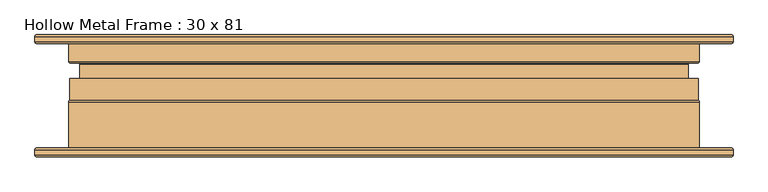
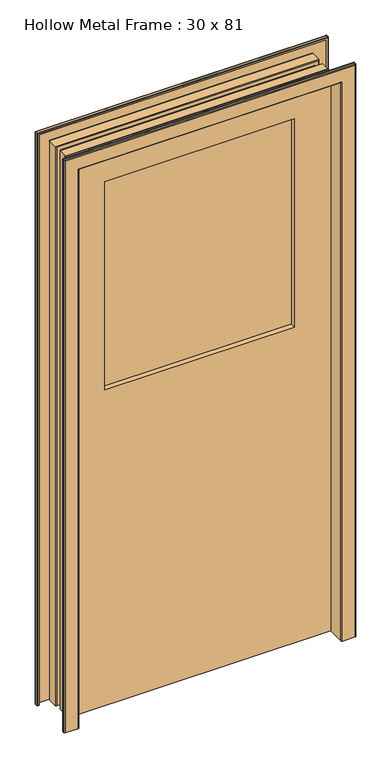
"""IFC4 building model written with IfcOpenShell, lengths in millimetres: door geometry, Hollow Metal Frame : 30 x 81."""

from ifc_helpers import new_model, si_unit, frame, origin, place, context, project, spatial, polyline, circle_curve, ellipse_curve, outline, extrude, source, transform, mapped, element, save
from ifc_brep_helpers import plane_surface, cylinder_surface, revolved_surface, advanced_brep


def hollow_metal_frame_30_x_81_1a9cdc0c(model_context):
    return source(origin(), model_context, "Body", "SolidModel", [
        extrude(outline(polyline([(330.2, 6.35), (330.2, -6.35), (-330.2, -6.35), (-330.2, 6.35), (330.2, 6.35)])), frame((0.0, 0.0, 1163.32), z_axis=(0.0, 0.0, 1.0), x_axis=(1.0, 0.0, 0.0)), (0.0, 0.0, 1.0), 767.08),
        extrude(outline(polyline([(2057.4, -457.2), (0.0, -457.2), (0.0, 457.2), (2057.4, 457.2), (2057.4, -457.2)]), holes=[polyline([(1930.4, -330.2), (1930.4, 330.2), (1163.32, 330.2), (1163.32, -330.2), (1930.4, -330.2)])]), frame((0.0, -25.4, 0.0), z_axis=(0.0, 1.0, 0.0), x_axis=(0.0, 0.0, 1.0)), (0.0, 0.0, 1.0), 50.8),
        advanced_brep(
        [(-505.42825, -76.2635, 0.0), (-500.0625, -76.2635, 0.0), (-500.0625, -77.81925, 0.0), (-505.42825, -77.81925, 0.0), (-506.44425, -78.83525, 0.0), (-506.44425, -86.36, 0.0), (-505.42825, -87.376, 0.0), (-459.77175, -87.376, 0.0), (-458.75575, -86.36, 0.0), (-458.75575, -8.98525, 0.0), (-456.184, -6.4135, 0.0), (-443.89675, -6.4135, 0.0), (-442.88075, -5.3975, 0.0), (-442.88075, 46.3931, 0.0), (-443.89675, 47.4091, 0.0), (-456.184, 47.4091, 0.0), (-458.75575, 49.98085, 0.0), (-458.75575, 86.2965, 0.0), (-459.77175, 87.3125, 0.0), (-505.42825, 87.3125, 0.0), (-506.44425, 86.2965, 0.0), (-506.44425, 78.77175, 0.0), (-505.42825, 77.75575, 0.0), (-500.0625, 77.75575, 0.0), (-500.0625, 76.2, 0.0), (-505.42825, 76.2, 0.0), (-508.0, 78.77175, 0.0), (-508.0, 86.2965, 0.0), (-505.42825, 88.86825, 0.0), (-459.77175, 88.86825, 0.0), (-457.2, 86.2965, 0.0), (-457.2, 49.98085, 0.0), (-456.184, 48.96485, 0.0), (-443.89675, 48.96485, 0.0), (-441.325, 46.3931, 0.0), (-441.325, -5.3975, 0.0), (-443.89675, -7.96925, 0.0), (-456.184, -7.96925, 0.0), (-457.2, -8.98525, 0.0), (-457.2, -86.36, 0.0), (-459.77175, -88.93175, 0.0), (-505.42825, -88.93175, 0.0), (-508.0, -86.36, 0.0), (-508.0, -78.83525, 0.0), (-508.0, -78.83525, 2108.2), (-505.42825, -76.2635, 2105.62825), (-508.0, -86.36, 2108.2), (-505.42825, -88.93175, 2105.62825), (-459.77175, -88.93175, 2059.97175), (459.77175, -88.93175, 2059.97175), (459.77175, -88.93175, 0.0), (505.42825, -88.93175, 0.0), (505.42825, -88.93175, 2105.62825), (-457.2, -86.36, 2057.4), (-457.2, -8.98525, 2057.4), (-456.184, -7.96925, 2056.384), (-443.89675, -7.96925, 2044.09675), (443.89675, -7.96925, 2044.09675), (443.89675, -7.96925, 0.0), (456.184, -7.96925, 0.0), (456.184, -7.96925, 2056.384), (-441.325, -5.3975, 2041.525), (-441.325, 46.3931, 2041.525), (-443.89675, 48.96485, 2044.09675), (-456.184, 48.96485, 2056.384), (456.184, 48.96485, 2056.384), (456.184, 48.96485, 0.0), (443.89675, 48.96485, 0.0), (443.89675, 48.96485, 2044.09675), (-457.2, 49.98085, 2057.4), (-457.2, 86.2965, 2057.4), (-459.77175, 88.86825, 2059.97175), (-505.42825, 88.86825, 2105.62825), (505.42825, 88.86825, 2105.62825), (505.42825, 88.86825, 0.0), (459.77175, 88.86825, 0.0), (459.77175, 88.86825, 2059.97175), (-508.0, 86.2965, 2108.2), (-508.0, 78.77175, 2108.2), (-505.42825, 76.2, 2105.62825), (-500.0625, 76.2, 2100.2625), (500.0625, 76.2, 2100.2625), (500.0625, 76.2, 0.0), (505.42825, 76.2, 0.0), (505.42825, 76.2, 2105.62825), (-500.0625, 77.75575, 2100.2625), (-505.42825, 77.75575, 2105.62825), (505.42825, 77.75575, 2105.62825), (505.42825, 77.75575, 0.0), (500.0625, 77.75575, 0.0), (500.0625, 77.75575, 2100.2625), (-506.44425, 78.77175, 2106.64425), (-506.44425, 86.2965, 2106.64425), (-505.42825, 87.3125, 2105.62825), (-459.77175, 87.3125, 2059.97175), (459.77175, 87.3125, 2059.97175), (459.77175, 87.3125, 0.0), (505.42825, 87.3125, 0.0), (505.42825, 87.3125, 2105.62825), (-458.75575, 86.2965, 2058.95575), (-458.75575, 49.98085, 2058.95575), (-456.184, 47.4091, 2056.384), (-443.89675, 47.4091, 2044.09675), (443.89675, 47.4091, 2044.09675), (443.89675, 47.4091, 0.0), (456.184, 47.4091, 0.0), (456.184, 47.4091, 2056.384), (-442.88075, 46.3931, 2043.08075), (-442.88075, -5.3975, 2043.08075), (-443.89675, -6.4135, 2044.09675), (-456.184, -6.4135, 2056.384), (456.184, -6.4135, 2056.384), (456.184, -6.4135, 0.0), (443.89675, -6.4135, 0.0), (443.89675, -6.4135, 2044.09675), (-458.75575, -8.98525, 2058.95575), (-458.75575, -86.36, 2058.95575), (-459.77175, -87.376, 2059.97175), (-505.42825, -87.376, 2105.62825), (505.42825, -87.376, 2105.62825), (505.42825, -87.376, 0.0), (459.77175, -87.376, 0.0), (459.77175, -87.376, 2059.97175), (-506.44425, -86.36, 2106.64425), (-506.44425, -78.83525, 2106.64425), (-505.42825, -77.81925, 2105.62825), (-500.0625, -77.81925, 2100.2625), (500.0625, -77.81925, 2100.2625), (500.0625, -77.81925, 0.0), (505.42825, -77.81925, 0.0), (505.42825, -77.81925, 2105.62825), (-500.0625, -76.2635, 2100.2625), (505.42825, -76.2635, 2105.62825), (505.42825, -76.2635, 0.0), (500.0625, -76.2635, 0.0), (500.0625, -76.2635, 2100.2625), (508.0, -78.83525, 2108.2), (508.0, -86.36, 2108.2), (457.2, -86.36, 2057.4), (457.2, -8.98525, 2057.4), (441.325, -5.3975, 2041.525), (441.325, 46.3931, 2041.525), (457.2, 49.98085, 2057.4), (457.2, 86.2965, 2057.4), (508.0, 86.2965, 2108.2), (508.0, 78.77175, 2108.2), (506.44425, 78.77175, 2106.64425), (506.44425, 86.2965, 2106.64425), (458.75575, 86.2965, 2058.95575), (458.75575, 49.98085, 2058.95575), (442.88075, 46.3931, 2043.08075), (442.88075, -5.3975, 2043.08075), (458.75575, -8.98525, 2058.95575), (458.75575, -86.36, 2058.95575), (506.44425, -86.36, 2106.64425), (506.44425, -78.83525, 2106.64425), (508.0, -78.83525, 0.0), (508.0, -86.36, 0.0), (457.2, -86.36, 0.0), (457.2, -8.98525, 0.0), (441.325, -5.3975, 0.0), (441.325, 46.3931, 0.0), (457.2, 49.98085, 0.0), (457.2, 86.2965, 0.0), (508.0, 86.2965, 0.0), (508.0, 78.77175, 0.0), (506.44425, 78.77175, 0.0), (506.44425, 86.2965, 0.0), (458.75575, 86.2965, 0.0), (458.75575, 49.98085, 0.0), (442.88075, 46.3931, 0.0), (442.88075, -5.3975, 0.0), (458.75575, -8.98525, 0.0), (458.75575, -86.36, 0.0), (506.44425, -86.36, 0.0), (506.44425, -78.83525, 0.0)],
        [
            (0, 1),
            (1, 2),
            (2, 3),
            (3, 4, circle_curve(frame((-505.42825, -78.83525, 0.0), z_axis=(0.0, 0.0, 1.0), x_axis=(0.0, 1.0, 0.0)), 1.016)),
            (4, 5),
            (5, 6, circle_curve(frame((-505.42825, -86.36, 0.0), z_axis=(0.0, 0.0, 1.0), x_axis=(0.0, 1.0, 0.0)), 1.016)),
            (6, 7),
            (7, 8, circle_curve(frame((-459.77175, -86.36, 0.0), z_axis=(0.0, 0.0, 1.0), x_axis=(0.0, 1.0, 0.0)), 1.016)),
            (8, 9),
            (9, 10, circle_curve(frame((-456.184, -8.98525, 0.0), z_axis=(0.0, 0.0, -1.0), x_axis=(0.0, 1.0, 0.0)), 2.57175)),
            (10, 11),
            (11, 12, circle_curve(frame((-443.89675, -5.3975, 0.0), z_axis=(0.0, 0.0, 1.0), x_axis=(0.0, 1.0, 0.0)), 1.016)),
            (12, 13),
            (13, 14, circle_curve(frame((-443.89675, 46.3931, 0.0), z_axis=(0.0, 0.0, 1.0), x_axis=(0.0, 1.0, 0.0)), 1.016)),
            (14, 15),
            (15, 16, circle_curve(frame((-456.184, 49.98085, 0.0), z_axis=(0.0, 0.0, -1.0), x_axis=(0.0, 1.0, 0.0)), 2.57175)),
            (16, 17),
            (17, 18, circle_curve(frame((-459.77175, 86.2965, 0.0), z_axis=(0.0, 0.0, 1.0), x_axis=(0.0, 1.0, 0.0)), 1.016)),
            (18, 19),
            (19, 20, circle_curve(frame((-505.42825, 86.2965, 0.0), z_axis=(0.0, 0.0, 1.0), x_axis=(0.0, 1.0, 0.0)), 1.016)),
            (20, 21),
            (21, 22, circle_curve(frame((-505.42825, 78.77175, 0.0), z_axis=(0.0, 0.0, 1.0), x_axis=(0.0, 1.0, 0.0)), 1.016)),
            (22, 23),
            (23, 24),
            (24, 25),
            (25, 26, circle_curve(frame((-505.42825, 78.77175, 0.0), z_axis=(0.0, 0.0, -1.0), x_axis=(0.0, 1.0, 0.0)), 2.57175)),
            (26, 27),
            (27, 28, circle_curve(frame((-505.42825, 86.2965, 0.0), z_axis=(0.0, 0.0, -1.0), x_axis=(0.0, 1.0, 0.0)), 2.57175)),
            (28, 29),
            (29, 30, circle_curve(frame((-459.77175, 86.2965, 0.0), z_axis=(0.0, 0.0, -1.0), x_axis=(0.0, 1.0, 0.0)), 2.57175)),
            (30, 31),
            (31, 32, circle_curve(frame((-456.184, 49.98085, 0.0), z_axis=(0.0, 0.0, 1.0), x_axis=(0.0, 1.0, 0.0)), 1.016)),
            (32, 33),
            (33, 34, circle_curve(frame((-443.89675, 46.3931, 0.0), z_axis=(0.0, 0.0, -1.0), x_axis=(0.0, 1.0, 0.0)), 2.57175)),
            (34, 35),
            (35, 36, circle_curve(frame((-443.89675, -5.3975, 0.0), z_axis=(0.0, 0.0, -1.0), x_axis=(0.0, 1.0, 0.0)), 2.57175)),
            (36, 37),
            (37, 38, circle_curve(frame((-456.184, -8.98525, 0.0), z_axis=(0.0, 0.0, 1.0), x_axis=(0.0, 1.0, 0.0)), 1.016)),
            (38, 39),
            (39, 40, circle_curve(frame((-459.77175, -86.36, 0.0), z_axis=(0.0, 0.0, -1.0), x_axis=(0.0, 1.0, 0.0)), 2.57175)),
            (40, 41),
            (41, 42, circle_curve(frame((-505.42825, -86.36, 0.0), z_axis=(0.0, 0.0, -1.0), x_axis=(0.0, 1.0, 0.0)), 2.57175)),
            (42, 43),
            (43, 0, circle_curve(frame((-505.42825, -78.83525, 0.0), z_axis=(0.0, 0.0, -1.0), x_axis=(0.0, 1.0, 0.0)), 2.57175)),
            (43, 44),
            (44, 45, ellipse_curve(frame((-505.42825, -78.83525, 2105.62825), z_axis=(-0.7071067811865475, 0.0, -0.7071067811865475), x_axis=(0.7071067811865474, 0.0, -0.7071067811865476)), 3.6370037, 2.57175)),
            (45, 0),
            (42, 46),
            (46, 44),
            (41, 47),
            (47, 46, ellipse_curve(frame((-505.42825, -86.36, 2105.62825), z_axis=(-0.7071067811865475, 0.0, -0.7071067811865475), x_axis=(0.7071067811865474, 0.0, -0.7071067811865476)), 3.6370037, 2.57175)),
            (40, 48),
            (48, 49),
            (49, 50),
            (50, 51),
            (51, 52),
            (52, 47),
            (39, 53),
            (53, 48, ellipse_curve(frame((-459.77175, -86.36, 2059.97175), z_axis=(-0.7071067811865475, 0.0, -0.7071067811865475), x_axis=(0.7071067811865474, 0.0, -0.7071067811865476)), 3.6370037, 2.57175)),
            (38, 54),
            (54, 53),
            (37, 55),
            (55, 54, ellipse_curve(frame((-456.184, -8.98525, 2056.384), z_axis=(0.7071067811865475, 0.0, 0.7071067811865475), x_axis=(-0.7071067811865474, 0.0, 0.7071067811865476)), 1.436841, 1.016)),
            (36, 56),
            (56, 57),
            (57, 58),
            (58, 59),
            (59, 60),
            (60, 55),
            (35, 61),
            (61, 56, ellipse_curve(frame((-443.89675, -5.3975, 2044.09675), z_axis=(-0.7071067811865475, 0.0, -0.7071067811865475), x_axis=(0.7071067811865474, 0.0, -0.7071067811865476)), 3.6370037, 2.57175)),
            (34, 62),
            (62, 61),
            (33, 63),
            (63, 62, ellipse_curve(frame((-443.89675, 46.3931, 2044.09675), z_axis=(-0.7071067811865475, 0.0, -0.7071067811865475), x_axis=(0.7071067811865474, 0.0, -0.7071067811865476)), 3.6370037, 2.57175)),
            (32, 64),
            (64, 65),
            (65, 66),
            (66, 67),
            (67, 68),
            (68, 63),
            (31, 69),
            (69, 64, ellipse_curve(frame((-456.184, 49.98085, 2056.384), z_axis=(0.7071067811865475, 0.0, 0.7071067811865475), x_axis=(-0.7071067811865474, 0.0, 0.7071067811865476)), 1.436841, 1.016)),
            (30, 70),
            (70, 69),
            (29, 71),
            (71, 70, ellipse_curve(frame((-459.77175, 86.2965, 2059.97175), z_axis=(-0.7071067811865475, 0.0, -0.7071067811865475), x_axis=(0.7071067811865474, 0.0, -0.7071067811865476)), 3.6370037, 2.57175)),
            (28, 72),
            (72, 73),
            (73, 74),
            (74, 75),
            (75, 76),
            (76, 71),
            (27, 77),
            (77, 72, ellipse_curve(frame((-505.42825, 86.2965, 2105.62825), z_axis=(-0.7071067811865475, 0.0, -0.7071067811865475), x_axis=(0.7071067811865474, 0.0, -0.7071067811865476)), 3.6370037, 2.57175)),
            (26, 78),
            (78, 77),
            (25, 79),
            (79, 78, ellipse_curve(frame((-505.42825, 78.77175, 2105.62825), z_axis=(-0.7071067811865475, 0.0, -0.7071067811865475), x_axis=(0.7071067811865474, 0.0, -0.7071067811865476)), 3.6370037, 2.57175)),
            (24, 80),
            (80, 81),
            (81, 82),
            (82, 83),
            (83, 84),
            (84, 79),
            (23, 85),
            (85, 80),
            (22, 86),
            (86, 87),
            (87, 88),
            (88, 89),
            (89, 90),
            (90, 85),
            (21, 91),
            (91, 86, ellipse_curve(frame((-505.42825, 78.77175, 2105.62825), z_axis=(0.7071067811865475, 0.0, 0.7071067811865475), x_axis=(-0.7071067811865474, 0.0, 0.7071067811865476)), 1.436841, 1.016)),
            (20, 92),
            (92, 91),
            (19, 93),
            (93, 92, ellipse_curve(frame((-505.42825, 86.2965, 2105.62825), z_axis=(0.7071067811865475, 0.0, 0.7071067811865475), x_axis=(-0.7071067811865474, 0.0, 0.7071067811865476)), 1.436841, 1.016)),
            (18, 94),
            (94, 95),
            (95, 96),
            (96, 97),
            (97, 98),
            (98, 93),
            (17, 99),
            (99, 94, ellipse_curve(frame((-459.77175, 86.2965, 2059.97175), z_axis=(0.7071067811865475, 0.0, 0.7071067811865475), x_axis=(-0.7071067811865474, 0.0, 0.7071067811865476)), 1.436841, 1.016)),
            (16, 100),
            (100, 99),
            (15, 101),
            (101, 100, ellipse_curve(frame((-456.184, 49.98085, 2056.384), z_axis=(-0.7071067811865475, 0.0, -0.7071067811865475), x_axis=(0.7071067811865474, 0.0, -0.7071067811865476)), 3.6370037, 2.57175)),
            (14, 102),
            (102, 103),
            (103, 104),
            (104, 105),
            (105, 106),
            (106, 101),
            (13, 107),
            (107, 102, ellipse_curve(frame((-443.89675, 46.3931, 2044.09675), z_axis=(0.7071067811865475, 0.0, 0.7071067811865475), x_axis=(-0.7071067811865474, 0.0, 0.7071067811865476)), 1.436841, 1.016)),
            (12, 108),
            (108, 107),
            (11, 109),
            (109, 108, ellipse_curve(frame((-443.89675, -5.3975, 2044.09675), z_axis=(0.7071067811865475, 0.0, 0.7071067811865475), x_axis=(-0.7071067811865474, 0.0, 0.7071067811865476)), 1.436841, 1.016)),
            (10, 110),
            (110, 111),
            (111, 112),
            (112, 113),
            (113, 114),
            (114, 109),
            (9, 115),
            (115, 110, ellipse_curve(frame((-456.184, -8.98525, 2056.384), z_axis=(-0.7071067811865475, 0.0, -0.7071067811865475), x_axis=(0.7071067811865474, 0.0, -0.7071067811865476)), 3.6370037, 2.57175)),
            (8, 116),
            (116, 115),
            (7, 117),
            (117, 116, ellipse_curve(frame((-459.77175, -86.36, 2059.97175), z_axis=(0.7071067811865475, 0.0, 0.7071067811865475), x_axis=(-0.7071067811865474, 0.0, 0.7071067811865476)), 1.436841, 1.016)),
            (6, 118),
            (118, 119),
            (119, 120),
            (120, 121),
            (121, 122),
            (122, 117),
            (5, 123),
            (123, 118, ellipse_curve(frame((-505.42825, -86.36, 2105.62825), z_axis=(0.7071067811865475, 0.0, 0.7071067811865475), x_axis=(-0.7071067811865474, 0.0, 0.7071067811865476)), 1.436841, 1.016)),
            (4, 124),
            (124, 123),
            (3, 125),
            (125, 124, ellipse_curve(frame((-505.42825, -78.83525, 2105.62825), z_axis=(0.7071067811865475, 0.0, 0.7071067811865475), x_axis=(-0.7071067811865474, 0.0, 0.7071067811865476)), 1.436841, 1.016)),
            (2, 126),
            (126, 127),
            (127, 128),
            (128, 129),
            (129, 130),
            (130, 125),
            (1, 131),
            (131, 126),
            (45, 132),
            (132, 133),
            (133, 134),
            (134, 135),
            (135, 131),
            (44, 136),
            (136, 132, ellipse_curve(frame((505.42825, -78.83525, 2105.62825), z_axis=(-0.7071067811865475, 0.0, 0.7071067811865475), x_axis=(-0.7071067811865476, 0.0, -0.7071067811865474)), 3.6370037, 2.57175)),
            (46, 137),
            (137, 136),
            (52, 137, ellipse_curve(frame((505.42825, -86.36, 2105.62825), z_axis=(-0.7071067811865475, 0.0, 0.7071067811865475), x_axis=(-0.7071067811865476, 0.0, -0.7071067811865474)), 3.6370037, 2.57175)),
            (53, 138),
            (138, 49, ellipse_curve(frame((459.77175, -86.36, 2059.97175), z_axis=(-0.7071067811865475, 0.0, 0.7071067811865475), x_axis=(-0.7071067811865476, 0.0, -0.7071067811865474)), 3.6370037, 2.57175)),
            (54, 139),
            (139, 138),
            (60, 139, ellipse_curve(frame((456.184, -8.98525, 2056.384), z_axis=(0.7071067811865475, 0.0, -0.7071067811865475), x_axis=(0.7071067811865476, 0.0, 0.7071067811865474)), 1.436841, 1.016)),
            (61, 140),
            (140, 57, ellipse_curve(frame((443.89675, -5.3975, 2044.09675), z_axis=(-0.7071067811865475, 0.0, 0.7071067811865475), x_axis=(-0.7071067811865476, 0.0, -0.7071067811865474)), 3.6370037, 2.57175)),
            (62, 141),
            (141, 140),
            (68, 141, ellipse_curve(frame((443.89675, 46.3931, 2044.09675), z_axis=(-0.7071067811865475, 0.0, 0.7071067811865475), x_axis=(-0.7071067811865476, 0.0, -0.7071067811865474)), 3.6370037, 2.57175)),
            (69, 142),
            (142, 65, ellipse_curve(frame((456.184, 49.98085, 2056.384), z_axis=(0.7071067811865475, 0.0, -0.7071067811865475), x_axis=(0.7071067811865476, 0.0, 0.7071067811865474)), 1.436841, 1.016)),
            (70, 143),
            (143, 142),
            (76, 143, ellipse_curve(frame((459.77175, 86.2965, 2059.97175), z_axis=(-0.7071067811865475, 0.0, 0.7071067811865475), x_axis=(-0.7071067811865476, 0.0, -0.7071067811865474)), 3.6370037, 2.57175)),
            (77, 144),
            (144, 73, ellipse_curve(frame((505.42825, 86.2965, 2105.62825), z_axis=(-0.7071067811865475, 0.0, 0.7071067811865475), x_axis=(-0.7071067811865476, 0.0, -0.7071067811865474)), 3.6370037, 2.57175)),
            (78, 145),
            (145, 144),
            (84, 145, ellipse_curve(frame((505.42825, 78.77175, 2105.62825), z_axis=(-0.7071067811865475, 0.0, 0.7071067811865475), x_axis=(-0.7071067811865476, 0.0, -0.7071067811865474)), 3.6370037, 2.57175)),
            (90, 81),
            (91, 146),
            (146, 87, ellipse_curve(frame((505.42825, 78.77175, 2105.62825), z_axis=(0.7071067811865475, 0.0, -0.7071067811865475), x_axis=(0.7071067811865476, 0.0, 0.7071067811865474)), 1.436841, 1.016)),
            (92, 147),
            (147, 146),
            (98, 147, ellipse_curve(frame((505.42825, 86.2965, 2105.62825), z_axis=(0.7071067811865475, 0.0, -0.7071067811865475), x_axis=(0.7071067811865476, 0.0, 0.7071067811865474)), 1.436841, 1.016)),
            (99, 148),
            (148, 95, ellipse_curve(frame((459.77175, 86.2965, 2059.97175), z_axis=(0.7071067811865475, 0.0, -0.7071067811865475), x_axis=(0.7071067811865476, 0.0, 0.7071067811865474)), 1.436841, 1.016)),
            (100, 149),
            (149, 148),
            (106, 149, ellipse_curve(frame((456.184, 49.98085, 2056.384), z_axis=(-0.7071067811865475, 0.0, 0.7071067811865475), x_axis=(-0.7071067811865476, 0.0, -0.7071067811865474)), 3.6370037, 2.57175)),
            (107, 150),
            (150, 103, ellipse_curve(frame((443.89675, 46.3931, 2044.09675), z_axis=(0.7071067811865475, 0.0, -0.7071067811865475), x_axis=(0.7071067811865476, 0.0, 0.7071067811865474)), 1.436841, 1.016)),
            (108, 151),
            (151, 150),
            (114, 151, ellipse_curve(frame((443.89675, -5.3975, 2044.09675), z_axis=(0.7071067811865475, 0.0, -0.7071067811865475), x_axis=(0.7071067811865476, 0.0, 0.7071067811865474)), 1.436841, 1.016)),
            (115, 152),
            (152, 111, ellipse_curve(frame((456.184, -8.98525, 2056.384), z_axis=(-0.7071067811865475, 0.0, 0.7071067811865475), x_axis=(-0.7071067811865476, 0.0, -0.7071067811865474)), 3.6370037, 2.57175)),
            (116, 153),
            (153, 152),
            (122, 153, ellipse_curve(frame((459.77175, -86.36, 2059.97175), z_axis=(0.7071067811865475, 0.0, -0.7071067811865475), x_axis=(0.7071067811865476, 0.0, 0.7071067811865474)), 1.436841, 1.016)),
            (123, 154),
            (154, 119, ellipse_curve(frame((505.42825, -86.36, 2105.62825), z_axis=(0.7071067811865475, 0.0, -0.7071067811865475), x_axis=(0.7071067811865476, 0.0, 0.7071067811865474)), 1.436841, 1.016)),
            (124, 155),
            (155, 154),
            (130, 155, ellipse_curve(frame((505.42825, -78.83525, 2105.62825), z_axis=(0.7071067811865475, 0.0, -0.7071067811865475), x_axis=(0.7071067811865476, 0.0, 0.7071067811865474)), 1.436841, 1.016)),
            (135, 127),
            (133, 156, circle_curve(frame((505.42825, -78.83525, 0.0), z_axis=(0.0, 0.0, -1.0), x_axis=(0.0, 1.0, 0.0)), 2.57175)),
            (156, 157),
            (157, 51, circle_curve(frame((505.42825, -86.36, 0.0), z_axis=(0.0, 0.0, -1.0), x_axis=(0.0, 1.0, 0.0)), 2.57175)),
            (50, 158, circle_curve(frame((459.77175, -86.36, 0.0), z_axis=(0.0, 0.0, -1.0), x_axis=(0.0, 1.0, 0.0)), 2.57175)),
            (158, 159),
            (159, 59, circle_curve(frame((456.184, -8.98525, 0.0), z_axis=(0.0, 0.0, 1.0), x_axis=(0.0, 1.0, 0.0)), 1.016)),
            (58, 160, circle_curve(frame((443.89675, -5.3975, 0.0), z_axis=(0.0, 0.0, -1.0), x_axis=(0.0, 1.0, 0.0)), 2.57175)),
            (160, 161),
            (161, 67, circle_curve(frame((443.89675, 46.3931, 0.0), z_axis=(0.0, 0.0, -1.0), x_axis=(0.0, 1.0, 0.0)), 2.57175)),
            (66, 162, circle_curve(frame((456.184, 49.98085, 0.0), z_axis=(0.0, 0.0, 1.0), x_axis=(0.0, 1.0, 0.0)), 1.016)),
            (162, 163),
            (163, 75, circle_curve(frame((459.77175, 86.2965, 0.0), z_axis=(0.0, 0.0, -1.0), x_axis=(0.0, 1.0, 0.0)), 2.57175)),
            (74, 164, circle_curve(frame((505.42825, 86.2965, 0.0), z_axis=(0.0, 0.0, -1.0), x_axis=(0.0, 1.0, 0.0)), 2.57175)),
            (164, 165),
            (165, 83, circle_curve(frame((505.42825, 78.77175, 0.0), z_axis=(0.0, 0.0, -1.0), x_axis=(0.0, 1.0, 0.0)), 2.57175)),
            (82, 89),
            (88, 166, circle_curve(frame((505.42825, 78.77175, 0.0), z_axis=(0.0, 0.0, 1.0), x_axis=(0.0, 1.0, 0.0)), 1.016)),
            (166, 167),
            (167, 97, circle_curve(frame((505.42825, 86.2965, 0.0), z_axis=(0.0, 0.0, 1.0), x_axis=(0.0, 1.0, 0.0)), 1.016)),
            (96, 168, circle_curve(frame((459.77175, 86.2965, 0.0), z_axis=(0.0, 0.0, 1.0), x_axis=(0.0, 1.0, 0.0)), 1.016)),
            (168, 169),
            (169, 105, circle_curve(frame((456.184, 49.98085, 0.0), z_axis=(0.0, 0.0, -1.0), x_axis=(0.0, 1.0, 0.0)), 2.57175)),
            (104, 170, circle_curve(frame((443.89675, 46.3931, 0.0), z_axis=(0.0, 0.0, 1.0), x_axis=(0.0, 1.0, 0.0)), 1.016)),
            (170, 171),
            (171, 113, circle_curve(frame((443.89675, -5.3975, 0.0), z_axis=(0.0, 0.0, 1.0), x_axis=(0.0, 1.0, 0.0)), 1.016)),
            (112, 172, circle_curve(frame((456.184, -8.98525, 0.0), z_axis=(0.0, 0.0, -1.0), x_axis=(0.0, 1.0, 0.0)), 2.57175)),
            (172, 173),
            (173, 121, circle_curve(frame((459.77175, -86.36, 0.0), z_axis=(0.0, 0.0, 1.0), x_axis=(0.0, 1.0, 0.0)), 1.016)),
            (120, 174, circle_curve(frame((505.42825, -86.36, 0.0), z_axis=(0.0, 0.0, 1.0), x_axis=(0.0, 1.0, 0.0)), 1.016)),
            (174, 175),
            (175, 129, circle_curve(frame((505.42825, -78.83525, 0.0), z_axis=(0.0, 0.0, 1.0), x_axis=(0.0, 1.0, 0.0)), 1.016)),
            (128, 134),
            (136, 156),
            (137, 157),
            (138, 158),
            (139, 159),
            (140, 160),
            (141, 161),
            (142, 162),
            (143, 163),
            (144, 164),
            (145, 165),
            (146, 166),
            (147, 167),
            (148, 168),
            (149, 169),
            (150, 170),
            (151, 171),
            (152, 172),
            (153, 173),
            (154, 174),
            (155, 175),
        ],
        [
            plane_surface(frame((-468.3125, 76.2, 0.0), z_axis=(0.0, 0.0, -1.0), x_axis=(1.0, 0.0, 0.0))),
            cylinder_surface(frame((-505.42825, -78.83525, 0.0), z_axis=(0.0, 0.0, -1.0), x_axis=(0.0, 1.0, 0.0)), 2.57175),
            plane_surface(frame((-508.0, -78.83525, 0.0), z_axis=(-1.0, 0.0, 0.0), x_axis=(0.0, 0.0, 1.0))),
            cylinder_surface(frame((-505.42825, -86.36, 0.0), z_axis=(0.0, 0.0, -1.0), x_axis=(0.0, 1.0, 0.0)), 2.57175),
            plane_surface(frame((-505.42825, -88.93175, 0.0), z_axis=(0.0, -1.0, 0.0), x_axis=(0.0, 0.0, 1.0))),
            cylinder_surface(frame((-459.77175, -86.36, 0.0), z_axis=(0.0, 0.0, -1.0), x_axis=(0.0, 1.0, 0.0)), 2.57175),
            plane_surface(frame((-457.2, -86.36, 0.0), z_axis=(1.0, 0.0, 0.0), x_axis=(0.0, 0.0, 1.0))),
            revolved_surface(polyline([(-456.184, -7.969250000000001, 2057.400000014587), (-456.184, -7.969250000000001, 0.0)]), (-456.184, -8.98525, 0.0), (0.0, 0.0, 1.0)),
            plane_surface(frame((-456.184, -7.96925, 0.0), z_axis=(0.0, -1.0, 0.0), x_axis=(0.0, 0.0, 1.0))),
            cylinder_surface(frame((-443.89675, -5.3975, 0.0), z_axis=(0.0, 0.0, -1.0), x_axis=(0.0, 1.0, 0.0)), 2.57175),
            plane_surface(frame((-441.325, -5.3975, 0.0), z_axis=(1.0, 0.0, 0.0), x_axis=(0.0, 0.0, 1.0))),
            cylinder_surface(frame((-443.89675, 46.3931, 0.0), z_axis=(0.0, 0.0, -1.0), x_axis=(0.0, 1.0, 0.0)), 2.57175),
            plane_surface(frame((-443.89675, 48.96485, 0.0), z_axis=(0.0, 1.0, 0.0), x_axis=(0.0, 0.0, 1.0))),
            revolved_surface(polyline([(-456.184, 50.996849999999995, 2057.400000014587), (-456.184, 50.996849999999995, 0.0)]), (-456.184, 49.98085, 0.0), (0.0, 0.0, 1.0)),
            plane_surface(frame((-457.2, 49.98085, 0.0), z_axis=(1.0, 0.0, 0.0), x_axis=(0.0, 0.0, 1.0))),
            cylinder_surface(frame((-459.77175, 86.2965, 0.0), z_axis=(0.0, 0.0, -1.0), x_axis=(0.0, 1.0, 0.0)), 2.57175),
            plane_surface(frame((-459.77175, 88.86825, 0.0), z_axis=(0.0, 1.0, 0.0), x_axis=(0.0, 0.0, 1.0))),
            cylinder_surface(frame((-505.42825, 86.2965, 0.0), z_axis=(0.0, 0.0, -1.0), x_axis=(0.0, 1.0, 0.0)), 2.57175),
            plane_surface(frame((-508.0, 86.2965, 0.0), z_axis=(-1.0, 0.0, 0.0), x_axis=(0.0, 0.0, 1.0))),
            cylinder_surface(frame((-505.42825, 78.77175, 0.0), z_axis=(0.0, 0.0, -1.0), x_axis=(0.0, 1.0, 0.0)), 2.57175),
            plane_surface(frame((-505.42825, 76.2, 0.0), z_axis=(0.0, -1.0, 0.0), x_axis=(0.0, 0.0, 1.0))),
            plane_surface(frame((-500.0625, 76.2, 0.0), z_axis=(1.0, 0.0, 0.0), x_axis=(0.0, 0.0, 1.0))),
            plane_surface(frame((-500.0625, 77.75575, 0.0), z_axis=(0.0, 1.0, 0.0), x_axis=(0.0, 0.0, 1.0))),
            revolved_surface(polyline([(-505.42825, 79.78775, 2106.644250014587), (-505.42825, 79.78775, 0.0)]), (-505.42825, 78.77175, 0.0), (0.0, 0.0, 1.0)),
            plane_surface(frame((-506.44425, 78.77175, 0.0), z_axis=(1.0, 0.0, 0.0), x_axis=(0.0, 0.0, 1.0))),
            revolved_surface(polyline([(-505.42825, 87.3125, 2106.644250014587), (-505.42825, 87.3125, 0.0)]), (-505.42825, 86.2965, 0.0), (0.0, 0.0, 1.0)),
            plane_surface(frame((-505.42825, 87.3125, 0.0), z_axis=(0.0, -1.0, 0.0), x_axis=(0.0, 0.0, 1.0))),
            revolved_surface(polyline([(-459.77175, 87.3125, 2060.987750014587), (-459.77175, 87.3125, 0.0)]), (-459.77175, 86.2965, 0.0), (0.0, 0.0, 1.0)),
            plane_surface(frame((-458.75575, 86.2965, 0.0), z_axis=(-1.0, 0.0, 0.0), x_axis=(0.0, 0.0, 1.0))),
            cylinder_surface(frame((-456.184, 49.98085, 0.0), z_axis=(0.0, 0.0, -1.0), x_axis=(0.0, 1.0, 0.0)), 2.57175),
            plane_surface(frame((-456.184, 47.4091, 0.0), z_axis=(0.0, -1.0, 0.0), x_axis=(0.0, 0.0, 1.0))),
            revolved_surface(polyline([(-443.89675, 47.409099999999995, 2045.1127500145867), (-443.89675, 47.409099999999995, 0.0)]), (-443.89675, 46.3931, 0.0), (0.0, 0.0, 1.0)),
            plane_surface(frame((-442.88075, 46.3931, 0.0), z_axis=(-1.0, 0.0, 0.0), x_axis=(0.0, 0.0, 1.0))),
            revolved_surface(polyline([(-443.89675, -4.3815, 2045.1127500145867), (-443.89675, -4.3815, 0.0)]), (-443.89675, -5.3975, 0.0), (0.0, 0.0, 1.0)),
            plane_surface(frame((-443.89675, -6.4135, 0.0), z_axis=(0.0, 1.0, 0.0), x_axis=(0.0, 0.0, 1.0))),
            cylinder_surface(frame((-456.184, -8.98525, 0.0), z_axis=(0.0, 0.0, -1.0), x_axis=(0.0, 1.0, 0.0)), 2.57175),
            plane_surface(frame((-458.75575, -8.98525, 0.0), z_axis=(-1.0, 0.0, 0.0), x_axis=(0.0, 0.0, 1.0))),
            revolved_surface(polyline([(-459.77175, -85.344, 2060.987750014587), (-459.77175, -85.344, 0.0)]), (-459.77175, -86.36, 0.0), (0.0, 0.0, 1.0)),
            plane_surface(frame((-459.77175, -87.376, 0.0), z_axis=(0.0, 1.0, 0.0), x_axis=(0.0, 0.0, 1.0))),
            revolved_surface(polyline([(-505.42825, -85.344, 2106.644250014587), (-505.42825, -85.344, 0.0)]), (-505.42825, -86.36, 0.0), (0.0, 0.0, 1.0)),
            plane_surface(frame((-506.44425, -86.36, 0.0), z_axis=(1.0, 0.0, 0.0), x_axis=(0.0, 0.0, 1.0))),
            revolved_surface(polyline([(-505.42825, -77.81925, 2106.644250014587), (-505.42825, -77.81925, 0.0)]), (-505.42825, -78.83525, 0.0), (0.0, 0.0, 1.0)),
            plane_surface(frame((-505.42825, -77.81925, 0.0), z_axis=(0.0, -1.0, 0.0), x_axis=(0.0, 0.0, 1.0))),
            plane_surface(frame((-500.0625, -77.81925, 0.0), z_axis=(1.0, 0.0, 0.0), x_axis=(0.0, 0.0, 1.0))),
            plane_surface(frame((-500.0625, -76.2635, 0.0), z_axis=(0.0, 1.0, 0.0), x_axis=(0.0, 0.0, 1.0))),
            cylinder_surface(frame((-468.3125, -78.83525, 2105.62825), z_axis=(-1.0, 0.0, 0.0), x_axis=(0.0, 1.0, 0.0)), 2.57175),
            plane_surface(frame((-508.0, -78.83525, 2108.2), z_axis=(0.0, 0.0, 1.0), x_axis=(1.0, 0.0, 0.0))),
            cylinder_surface(frame((-468.3125, -86.36, 2105.62825), z_axis=(-1.0, 0.0, 0.0), x_axis=(0.0, 1.0, 0.0)), 2.57175),
            cylinder_surface(frame((-468.3125, -86.36, 2059.97175), z_axis=(-1.0, 0.0, 0.0), x_axis=(0.0, 1.0, 0.0)), 2.57175),
            plane_surface(frame((-457.2, -86.36, 2057.4), z_axis=(0.0, 0.0, -1.0), x_axis=(1.0, 0.0, 0.0))),
            revolved_surface(polyline([(457.20000001458686, -7.969250000000001, 2056.384), (-457.20000001458686, -7.969250000000001, 2056.384)]), (-468.3125, -8.98525, 2056.384), (1.0, 0.0, 0.0)),
            cylinder_surface(frame((-468.3125, -5.3975, 2044.09675), z_axis=(-1.0, 0.0, 0.0), x_axis=(0.0, 1.0, 0.0)), 2.57175),
            plane_surface(frame((-441.325, -5.3975, 2041.525), z_axis=(0.0, 0.0, -1.0), x_axis=(1.0, 0.0, 0.0))),
            cylinder_surface(frame((-468.3125, 46.3931, 2044.09675), z_axis=(-1.0, 0.0, 0.0), x_axis=(0.0, 1.0, 0.0)), 2.57175),
            revolved_surface(polyline([(457.20000001458686, 50.996849999999995, 2056.384), (-457.20000001458686, 50.996849999999995, 2056.384)]), (-468.3125, 49.98085, 2056.384), (1.0, 0.0, 0.0)),
            plane_surface(frame((-457.2, 49.98085, 2057.4), z_axis=(0.0, 0.0, -1.0), x_axis=(1.0, 0.0, 0.0))),
            cylinder_surface(frame((-468.3125, 86.2965, 2059.97175), z_axis=(-1.0, 0.0, 0.0), x_axis=(0.0, 1.0, 0.0)), 2.57175),
            cylinder_surface(frame((-468.3125, 86.2965, 2105.62825), z_axis=(-1.0, 0.0, 0.0), x_axis=(0.0, 1.0, 0.0)), 2.57175),
            plane_surface(frame((-508.0, 86.2965, 2108.2), z_axis=(0.0, 0.0, 1.0), x_axis=(1.0, 0.0, 0.0))),
            cylinder_surface(frame((-468.3125, 78.77175, 2105.62825), z_axis=(-1.0, 0.0, 0.0), x_axis=(0.0, 1.0, 0.0)), 2.57175),
            plane_surface(frame((-500.0625, 76.2, 2100.2625), z_axis=(0.0, 0.0, -1.0), x_axis=(1.0, 0.0, 0.0))),
            revolved_surface(polyline([(506.4442500145868, 79.78775, 2105.62825), (-506.4442500145868, 79.78775, 2105.62825)]), (-468.3125, 78.77175, 2105.62825), (1.0, 0.0, 0.0)),
            plane_surface(frame((-506.44425, 78.77175, 2106.64425), z_axis=(0.0, 0.0, -1.0), x_axis=(1.0, 0.0, 0.0))),
            revolved_surface(polyline([(506.4442500145868, 87.3125, 2105.62825), (-506.4442500145868, 87.3125, 2105.62825)]), (-468.3125, 86.2965, 2105.62825), (1.0, 0.0, 0.0)),
            revolved_surface(polyline([(460.7877500145869, 87.3125, 2059.97175), (-460.78775001458683, 87.3125, 2059.97175)]), (-468.3125, 86.2965, 2059.97175), (1.0, 0.0, 0.0)),
            plane_surface(frame((-458.75575, 86.2965, 2058.95575), z_axis=(0.0, 0.0, 1.0), x_axis=(1.0, 0.0, 0.0))),
            cylinder_surface(frame((-468.3125, 49.98085, 2056.384), z_axis=(-1.0, 0.0, 0.0), x_axis=(0.0, 1.0, 0.0)), 2.57175),
            revolved_surface(polyline([(444.9127500145869, 47.409099999999995, 2044.09675), (-444.91275001458683, 47.409099999999995, 2044.09675)]), (-468.3125, 46.3931, 2044.09675), (1.0, 0.0, 0.0)),
            plane_surface(frame((-442.88075, 46.3931, 2043.08075), z_axis=(0.0, 0.0, 1.0), x_axis=(1.0, 0.0, 0.0))),
            revolved_surface(polyline([(444.9127500145869, -4.3815, 2044.09675), (-444.91275001458683, -4.3815, 2044.09675)]), (-468.3125, -5.3975, 2044.09675), (1.0, 0.0, 0.0)),
            cylinder_surface(frame((-468.3125, -8.98525, 2056.384), z_axis=(-1.0, 0.0, 0.0), x_axis=(0.0, 1.0, 0.0)), 2.57175),
            plane_surface(frame((-458.75575, -8.98525, 2058.95575), z_axis=(0.0, 0.0, 1.0), x_axis=(1.0, 0.0, 0.0))),
            revolved_surface(polyline([(460.7877500145869, -85.344, 2059.97175), (-460.78775001458683, -85.344, 2059.97175)]), (-468.3125, -86.36, 2059.97175), (1.0, 0.0, 0.0)),
            revolved_surface(polyline([(506.4442500145868, -85.344, 2105.62825), (-506.4442500145868, -85.344, 2105.62825)]), (-468.3125, -86.36, 2105.62825), (1.0, 0.0, 0.0)),
            plane_surface(frame((-506.44425, -86.36, 2106.64425), z_axis=(0.0, 0.0, -1.0), x_axis=(1.0, 0.0, 0.0))),
            revolved_surface(polyline([(506.4442500145868, -77.81925, 2105.62825), (-506.4442500145868, -77.81925, 2105.62825)]), (-468.3125, -78.83525, 2105.62825), (1.0, 0.0, 0.0)),
            plane_surface(frame((-500.0625, -77.81925, 2100.2625), z_axis=(0.0, 0.0, -1.0), x_axis=(1.0, 0.0, 0.0))),
            plane_surface(frame((468.3125, 76.2, 0.0), z_axis=(0.0, 0.0, -1.0), x_axis=(-1.0, 0.0, 0.0))),
            cylinder_surface(frame((505.42825, -78.83525, 2068.5125), z_axis=(0.0, 0.0, 1.0), x_axis=(0.0, 1.0, 0.0)), 2.57175),
            plane_surface(frame((508.0, -78.83525, 2108.2), z_axis=(1.0, 0.0, 0.0), x_axis=(0.0, 0.0, -1.0))),
            cylinder_surface(frame((505.42825, -86.36, 2068.5125), z_axis=(0.0, 0.0, 1.0), x_axis=(0.0, 1.0, 0.0)), 2.57175),
            cylinder_surface(frame((459.77175, -86.36, 2068.5125), z_axis=(0.0, 0.0, 1.0), x_axis=(0.0, 1.0, 0.0)), 2.57175),
            plane_surface(frame((457.2, -86.36, 2057.4), z_axis=(-1.0, 0.0, 0.0), x_axis=(0.0, 0.0, -1.0))),
            revolved_surface(polyline([(456.184, -7.969250000000001, 0.0), (456.184, -7.969250000000001, 2057.400000014587)]), (456.184, -8.98525, 2068.5125), (0.0, 0.0, -1.0)),
            cylinder_surface(frame((443.89675, -5.3975, 2068.5125), z_axis=(0.0, 0.0, 1.0), x_axis=(0.0, 1.0, 0.0)), 2.57175),
            plane_surface(frame((441.325, -5.3975, 2041.525), z_axis=(-1.0, 0.0, 0.0), x_axis=(0.0, 0.0, -1.0))),
            cylinder_surface(frame((443.89675, 46.3931, 2068.5125), z_axis=(0.0, 0.0, 1.0), x_axis=(0.0, 1.0, 0.0)), 2.57175),
            revolved_surface(polyline([(456.184, 50.996849999999995, 0.0), (456.184, 50.996849999999995, 2057.400000014587)]), (456.184, 49.98085, 2068.5125), (0.0, 0.0, -1.0)),
            plane_surface(frame((457.2, 49.98085, 2057.4), z_axis=(-1.0, 0.0, 0.0), x_axis=(0.0, 0.0, -1.0))),
            cylinder_surface(frame((459.77175, 86.2965, 2068.5125), z_axis=(0.0, 0.0, 1.0), x_axis=(0.0, 1.0, 0.0)), 2.57175),
            cylinder_surface(frame((505.42825, 86.2965, 2068.5125), z_axis=(0.0, 0.0, 1.0), x_axis=(0.0, 1.0, 0.0)), 2.57175),
            plane_surface(frame((508.0, 86.2965, 2108.2), z_axis=(1.0, 0.0, 0.0), x_axis=(0.0, 0.0, -1.0))),
            cylinder_surface(frame((505.42825, 78.77175, 2068.5125), z_axis=(0.0, 0.0, 1.0), x_axis=(0.0, 1.0, 0.0)), 2.57175),
            plane_surface(frame((500.0625, 76.2, 2100.2625), z_axis=(-1.0, 0.0, 0.0), x_axis=(0.0, 0.0, -1.0))),
            revolved_surface(polyline([(505.42825, 79.78775, 0.0), (505.42825, 79.78775, 2106.644250014587)]), (505.42825, 78.77175, 2068.5125), (0.0, 0.0, -1.0)),
            plane_surface(frame((506.44425, 78.77175, 2106.64425), z_axis=(-1.0, 0.0, 0.0), x_axis=(0.0, 0.0, -1.0))),
            revolved_surface(polyline([(505.42825, 87.3125, 0.0), (505.42825, 87.3125, 2106.644250014587)]), (505.42825, 86.2965, 2068.5125), (0.0, 0.0, -1.0)),
            revolved_surface(polyline([(459.77175, 87.3125, 0.0), (459.77175, 87.3125, 2060.987750014587)]), (459.77175, 86.2965, 2068.5125), (0.0, 0.0, -1.0)),
            plane_surface(frame((458.75575, 86.2965, 2058.95575), z_axis=(1.0, 0.0, 0.0), x_axis=(0.0, 0.0, -1.0))),
            cylinder_surface(frame((456.184, 49.98085, 2068.5125), z_axis=(0.0, 0.0, 1.0), x_axis=(0.0, 1.0, 0.0)), 2.57175),
            revolved_surface(polyline([(443.89675, 47.409099999999995, 0.0), (443.89675, 47.409099999999995, 2045.1127500145867)]), (443.89675, 46.3931, 2068.5125), (0.0, 0.0, -1.0)),
            plane_surface(frame((442.88075, 46.3931, 2043.08075), z_axis=(1.0, 0.0, 0.0), x_axis=(0.0, 0.0, -1.0))),
            revolved_surface(polyline([(443.89675, -4.3815, 0.0), (443.89675, -4.3815, 2045.1127500145867)]), (443.89675, -5.3975, 2068.5125), (0.0, 0.0, -1.0)),
            cylinder_surface(frame((456.184, -8.98525, 2068.5125), z_axis=(0.0, 0.0, 1.0), x_axis=(0.0, 1.0, 0.0)), 2.57175),
            plane_surface(frame((458.75575, -8.98525, 2058.95575), z_axis=(1.0, 0.0, 0.0), x_axis=(0.0, 0.0, -1.0))),
            revolved_surface(polyline([(459.77175, -85.344, 0.0), (459.77175, -85.344, 2060.987750014587)]), (459.77175, -86.36, 2068.5125), (0.0, 0.0, -1.0)),
            revolved_surface(polyline([(505.42825, -85.344, 0.0), (505.42825, -85.344, 2106.644250014587)]), (505.42825, -86.36, 2068.5125), (0.0, 0.0, -1.0)),
            plane_surface(frame((506.44425, -86.36, 2106.64425), z_axis=(-1.0, 0.0, 0.0), x_axis=(0.0, 0.0, -1.0))),
            revolved_surface(polyline([(505.42825, -77.81925, 0.0), (505.42825, -77.81925, 2106.644250014587)]), (505.42825, -78.83525, 2068.5125), (0.0, 0.0, -1.0)),
            plane_surface(frame((500.0625, -77.81925, 2100.2625), z_axis=(-1.0, 0.0, 0.0), x_axis=(0.0, 0.0, -1.0))),
        ],
        [
            (0, [[1, 2, 3, 4, 5, 6, 7, 8, 9, 10, 11, 12, 13, 14, 15, 16, 17, 18, 19, 20, 21, 22, 23, 24, 25, 26, 27, 28, 29, 30, 31, 32, 33, 34, 35, 36, 37, 38, 39, 40, 41, 42, 43, 44]]),
            (1, [[45, 46, 47, -44]]),
            (2, [[48, 49, -45, -43]]),
            (3, [[50, 51, -48, -42]]),
            (4, [[52, 53, 54, 55, 56, 57, -50, -41]]),
            (5, [[58, 59, -52, -40]]),
            (6, [[60, 61, -58, -39]]),
            (7, [[62, 63, -60, -38]]),
            (8, [[64, 65, 66, 67, 68, 69, -62, -37]]),
            (9, [[70, 71, -64, -36]]),
            (10, [[72, 73, -70, -35]]),
            (11, [[74, 75, -72, -34]]),
            (12, [[76, 77, 78, 79, 80, 81, -74, -33]]),
            (13, [[82, 83, -76, -32]]),
            (14, [[84, 85, -82, -31]]),
            (15, [[86, 87, -84, -30]]),
            (16, [[88, 89, 90, 91, 92, 93, -86, -29]]),
            (17, [[94, 95, -88, -28]]),
            (18, [[96, 97, -94, -27]]),
            (19, [[98, 99, -96, -26]]),
            (20, [[100, 101, 102, 103, 104, 105, -98, -25]]),
            (21, [[106, 107, -100, -24]]),
            (22, [[108, 109, 110, 111, 112, 113, -106, -23]]),
            (23, [[114, 115, -108, -22]]),
            (24, [[116, 117, -114, -21]]),
            (25, [[118, 119, -116, -20]]),
            (26, [[120, 121, 122, 123, 124, 125, -118, -19]]),
            (27, [[126, 127, -120, -18]]),
            (28, [[128, 129, -126, -17]]),
            (29, [[130, 131, -128, -16]]),
            (30, [[132, 133, 134, 135, 136, 137, -130, -15]]),
            (31, [[138, 139, -132, -14]]),
            (32, [[140, 141, -138, -13]]),
            (33, [[142, 143, -140, -12]]),
            (34, [[144, 145, 146, 147, 148, 149, -142, -11]]),
            (35, [[150, 151, -144, -10]]),
            (36, [[152, 153, -150, -9]]),
            (37, [[154, 155, -152, -8]]),
            (38, [[156, 157, 158, 159, 160, 161, -154, -7]]),
            (39, [[162, 163, -156, -6]]),
            (40, [[164, 165, -162, -5]]),
            (41, [[166, 167, -164, -4]]),
            (42, [[168, 169, 170, 171, 172, 173, -166, -3]]),
            (43, [[174, 175, -168, -2]]),
            (44, [[-47, 176, 177, 178, 179, 180, -174, -1]]),
            (45, [[181, 182, -176, -46]]),
            (46, [[183, 184, -181, -49]]),
            (47, [[-57, 185, -183, -51]]),
            (48, [[186, 187, -53, -59]]),
            (49, [[188, 189, -186, -61]]),
            (50, [[-69, 190, -188, -63]]),
            (51, [[191, 192, -65, -71]]),
            (52, [[193, 194, -191, -73]]),
            (53, [[-81, 195, -193, -75]]),
            (54, [[196, 197, -77, -83]]),
            (55, [[198, 199, -196, -85]]),
            (56, [[-93, 200, -198, -87]]),
            (57, [[201, 202, -89, -95]]),
            (58, [[203, 204, -201, -97]]),
            (59, [[-105, 205, -203, -99]]),
            (60, [[-113, 206, -101, -107]]),
            (61, [[207, 208, -109, -115]]),
            (62, [[209, 210, -207, -117]]),
            (63, [[-125, 211, -209, -119]]),
            (64, [[212, 213, -121, -127]]),
            (65, [[214, 215, -212, -129]]),
            (66, [[-137, 216, -214, -131]]),
            (67, [[217, 218, -133, -139]]),
            (68, [[219, 220, -217, -141]]),
            (69, [[-149, 221, -219, -143]]),
            (70, [[222, 223, -145, -151]]),
            (71, [[224, 225, -222, -153]]),
            (72, [[-161, 226, -224, -155]]),
            (73, [[227, 228, -157, -163]]),
            (74, [[229, 230, -227, -165]]),
            (75, [[-173, 231, -229, -167]]),
            (76, [[-180, 232, -169, -175]]),
            (77, [[233, 234, 235, -55, 236, 237, 238, -67, 239, 240, 241, -79, 242, 243, 244, -91, 245, 246, 247, -103, 248, -111, 249, 250, 251, -123, 252, 253, 254, -135, 255, 256, 257, -147, 258, 259, 260, -159, 261, 262, 263, -171, 264, -178]]),
            (78, [[265, -233, -177, -182]]),
            (79, [[266, -234, -265, -184]]),
            (80, [[-56, -235, -266, -185]]),
            (81, [[267, -236, -54, -187]]),
            (82, [[268, -237, -267, -189]]),
            (83, [[-68, -238, -268, -190]]),
            (84, [[269, -239, -66, -192]]),
            (85, [[270, -240, -269, -194]]),
            (86, [[-80, -241, -270, -195]]),
            (87, [[271, -242, -78, -197]]),
            (88, [[272, -243, -271, -199]]),
            (89, [[-92, -244, -272, -200]]),
            (90, [[273, -245, -90, -202]]),
            (91, [[274, -246, -273, -204]]),
            (92, [[-104, -247, -274, -205]]),
            (93, [[-112, -248, -102, -206]]),
            (94, [[275, -249, -110, -208]]),
            (95, [[276, -250, -275, -210]]),
            (96, [[-124, -251, -276, -211]]),
            (97, [[277, -252, -122, -213]]),
            (98, [[278, -253, -277, -215]]),
            (99, [[-136, -254, -278, -216]]),
            (100, [[279, -255, -134, -218]]),
            (101, [[280, -256, -279, -220]]),
            (102, [[-148, -257, -280, -221]]),
            (103, [[281, -258, -146, -223]]),
            (104, [[282, -259, -281, -225]]),
            (105, [[-160, -260, -282, -226]]),
            (106, [[283, -261, -158, -228]]),
            (107, [[284, -262, -283, -230]]),
            (108, [[-172, -263, -284, -231]]),
            (109, [[-179, -264, -170, -232]]),
        ],
    ),
    ])


if __name__ == "__main__":
    model = new_model("IFC4")
    model_context = context("Model", 3, world=origin())
    ifc_project = project(units=[si_unit("LENGTHUNIT", "METRE", prefix="MILLI")], contexts=[model_context])
    site = spatial("IfcSite", under=ifc_project)
    building = spatial("IfcBuilding", under=site)
    placement = place(None, origin())
    hollow_metal_frame_30_x_81_shape = hollow_metal_frame_30_x_81_1a9cdc0c(model_context)
    element("IfcDoor", 1, ObjectType="Hollow Metal Frame : 30 x 81", at=placement, inside=building, context=model_context, shape_type="MappedRepresentation", body=[
        mapped(hollow_metal_frame_30_x_81_shape, transform((0.0, 0.0, 0.0), x_axis=(1.0, 0.0, 0.0), y_axis=(0.0, 1.0, 0.0), z_axis=(0.0, 0.0, 1.0))),
    ])
    save(model, "model.ifc")

# Revit data of these elements
# Type "Hollow Metal Frame : 30 x 81"
#   Type Mark = "i"
#   Product Page URL = ""
#   Product Name = ""
#   Product Documentation Link = ""
#   Material = ""
#   DS_Hardware_Set_(SFT) = ""
#   DS_Frame_Type_(SFT) = ""
#   DS_Fire_Rating_(SFT) = ""
#   DS_Door_Type_(SFT) = ""
#   Analytic Construction = "<None>"
#   inset = 0' - 5"
#   Window Height = 2' - 6.2"
#   Frame Projection Ext. = 0' - 1"
#   Frame Projection Int. = 0' - 1"
#   Frame Width = 0' - 3"
#   Height = 6' - 9"
#   Width = 3' - 0"
#   Non-Kerfed = yes
#   Kerfed = no
#   Hollow Metal Casing = Metal-Dunbarton_Doors-White
#   Glass Material = none
#   Flush Door = Metal-Dunbarton_Doors-Aluminum
#   DS_Frame_Material_(SFT) = none
#   DS_Door_Material_(SFT) = EXISTING DOOR
#   URL = ""
#   Model = ""
#   Manufacturer = ""
#   Function = (empty or 0)
#   Wall Closure = (empty or 0)
#   Description = (empty or 0)
# Element 1 (IfcDoor, "Hollow Metal Frame : 30 x 81")
#   Materials on its faces: "EXISTING DOOR"
# Materials
#   "Metal-Dunbarton_Doors-White": class "Miscellaneous", colour RGB 230 233 236, transparency 0
#   "Metal-Dunbarton_Doors-Aluminum": class "System", colour RGB 143 142 141, transparency 0
#   "EXISTING DOOR": class "Generic", colour RGB 120 120 120, transparency 0, Cost = 0
